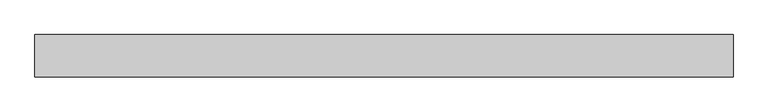
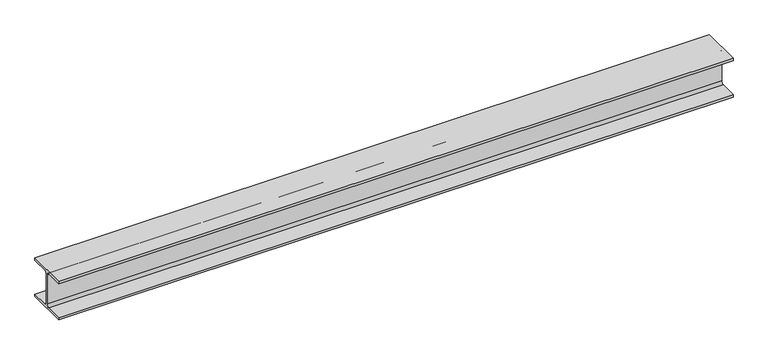
"""IFC4 building model written with IfcOpenShell, lengths in millimetres: beam geometry, 0912_Steel Framing_H-KSD3502 : H_SB_ASB_H-200x200x8x12."""

from ifc_helpers import new_model, si_unit, point, frame, frame_2d, origin, place, context, project, spatial, polyline, circle_curve, trimmed, segment, composite_curve, outline, extrude, source, transform, mapped, element, save


def beam_b68f9391(model_context):
    return source(origin(), model_context, "Body", "SweptSolid", [
        extrude(outline(composite_curve([segment(polyline([(100.0, -88.0), (100.0, -100.0), (-100.0, -100.0), (-100.0, -88.0), (-17.0, -88.0)]), True, "CONTINUOUS"), segment(trimmed(circle_curve(frame_2d((-17.0, -75.0)), 13.0), [point((-17.0, -88.0))], [point((-4.0, -75.0))], True, "CARTESIAN"), True, "CONTINUOUS"), segment(polyline([(-4.0, -75.0), (-4.0, 75.0)]), True, "CONTINUOUS"), segment(trimmed(circle_curve(frame_2d((-17.0, 75.0)), 13.0), [point((-4.0, 75.0))], [point((-17.0, 88.0))], True, "CARTESIAN"), True, "CONTINUOUS"), segment(polyline([(-17.0, 88.0), (-100.0, 88.0), (-100.0, 100.0), (100.0, 100.0), (100.0, 88.0), (17.0, 88.0)]), True, "CONTINUOUS"), segment(trimmed(circle_curve(frame_2d((17.0, 75.0)), 13.0), [point((17.0, 88.0))], [point((4.0, 75.0))], True, "CARTESIAN"), True, "CONTINUOUS"), segment(polyline([(4.0, 75.0), (4.0, -75.0)]), True, "CONTINUOUS"), segment(trimmed(circle_curve(frame_2d((17.0, -75.0)), 13.0), [point((4.0, -75.0))], [point((17.0, -88.0))], True, "CARTESIAN"), True, "CONTINUOUS"), segment(polyline([(17.0, -88.0), (100.0, -88.0)]), True, "CONTINUOUS")], self_intersect=False)), frame((-1713.3400783, 0.0, 0.0), z_axis=(1.0, 0.0, 0.0), x_axis=(0.0, 1.0, 0.0)), (0.0, 0.0, 1.0), 3299.2628363),
    ])


if __name__ == "__main__":
    model = new_model("IFC4")
    model_context = context("Model", 3, world=origin())
    ifc_project = project(units=[si_unit("LENGTHUNIT", "METRE", prefix="MILLI")], contexts=[model_context])
    site = spatial("IfcSite", under=ifc_project)
    building = spatial("IfcBuilding", under=site)
    placement = place(None, origin())
    beam_shape = beam_b68f9391(model_context)
    element("IfcBeam", 1, ObjectType="0912_Steel Framing_H-KSD3502 : H_SB_ASB_H-200x200x8x12", at=placement, inside=building, context=model_context, shape_type="MappedRepresentation", body=[
        mapped(beam_shape, transform((0.0, 0.0, 0.0), x_axis=(1.0, 0.0, 0.0), y_axis=(0.0, 1.0, 0.0), z_axis=(0.0, 0.0, 1.0))),
    ])
    save(model, "model.ifc")

# Revit data of these elements
# Type "0912_Steel Framing_H-KSD3502 : H_SB_ASB_H-200x200x8x12"
#   H_WM Code_1 = "S01AA002-00001 | Main Steel Structure Fabrication Work | Shelter/Building | Medium Steel - Standard (90KG/M>Weight≥30KG/M) | Material: (   )"
#   H_WM Code_2 = "S03AA028-00001 | Main Steel Structure Erection Work | Shelter/Building | Medium Steel (90KG/M>Weight≥30KG/M) | Material: (   )"
#   H_WM Code_3 = "S01AA010-00001 | Main Steel Structure Fabrication Work | Shelter/Building | Steel Painting/Coating | for Non-Fireproofed Steel Surface, Surface Preparation, Primer, Second & Final Coat | Material: (   )"
#   H_Q'ty Cal Type Tag = "SB-Q2"
#   Width = 20.0 cm
#   Web Thickness = 0.8 cm
#   Web Fillet = 1.3 cm
#   Warping Constant = 141000.0 cm⁶
#   W = 0
#   Torsional Moment of Inertia = 26.2485 cm⁴
#   Section Area = 63.53 cm²
#   Plastic Modulus weak axis = 244.0 cm³
#   Plastic Modulus strong axis = 525.0 cm³
#   Perimeter = 1.16 m²/m
#   Nominal Weight = 49.90 kgf/m
#   Moment of Inertia weak axis = 1600.00 cm⁴
#   Moment of Inertia strong axis = 4720.00 cm⁴
#   Height = 20.0 cm
#   Flange Thickness = 1.2 cm
#   Elastic Modulus weak axis = 160.0 cm³
#   Elastic Modulus strong axis = 472.0 cm³
#   Centroid Vertical = 10.0 cm
#   Centroid Horizontal = 10.0 cm
#   Ix = 47200000
#   Length [instance default] = 1.5240 m
#   Zx = 525000
#   b = 0.2000 m
#   h = 0.2000 m
#   r = 0.0130 m
#   s = 0.0080 m
#   t = 0.0120 m
#   A = 0.006353 m²
#   Structural Material [instance default] = Steel, 45-345
#   Assembly Code = ""
# Element 1 (IfcBeam, "0912_Steel Framing_H-KSD3502 : H_SB_ASB_H-200x200x8x12")
#   Structural Material = none
# Materials
#   "Steel, 45-345": class "Metal", colour RGB 189 187 185, transparency 0, Description = "Steel 345 MPa", Cost = 0
